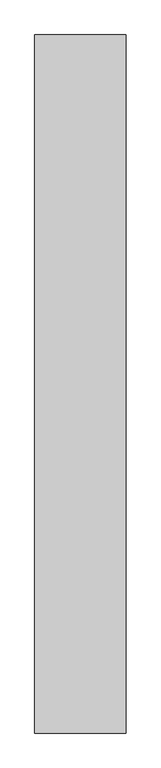
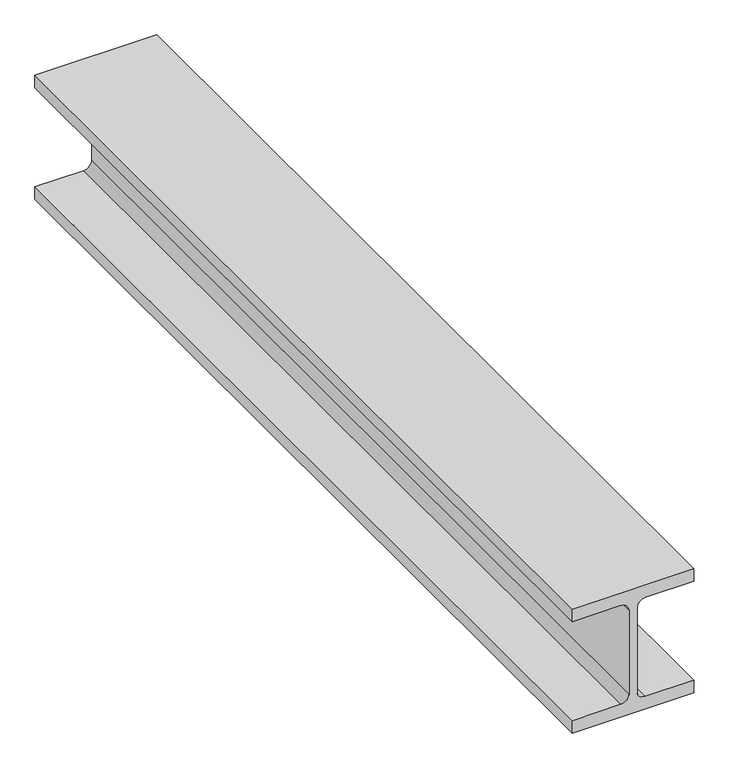
"""IFC4 building model written with IfcOpenShell, lengths in millimetres: proxy geometry, Structure061 17491 : Structure061 17491."""

import ifcopenshell
import ifcopenshell.guid

model = None  # the IFC model being written
_history = None  # IfcOwnerHistory: only IFC2X3 demands one
_inside = {}  # id of a spatial element -> (the spatial element, [elements in it])
_under = {}  # id of a project, library or spatial element -> (it, [spatial elements below it])
_declared = {}  # id of a project -> (the project, [libraries it declares])
_typed = {}  # id of a type object -> (the type object, [elements of that type])
_made_of = {}  # id of a material, layer set ... -> (it, [elements and type objects made of it])


def new_model(schema):
    """Start an empty IFC model of exactly this schema.

    Asked for "IFC4X3", IfcOpenShell would pick the latest addendum, in which some entities
    have other attributes; the version numbers below select the first issue.
    IFC2X3 requires an IfcOwnerHistory on every rooted entity: one is made here for all.
    """
    global model, _history
    if schema == "IFC4X3":
        model = ifcopenshell.file(schema_version=(4, 3, 0, 0))
    else:
        model = ifcopenshell.file(schema=schema)
    _inside.clear()
    _under.clear()
    _declared.clear()
    _typed.clear()
    _made_of.clear()
    _history = None
    if model.schema == "IFC2X3":
        org = make("IfcOrganization", Name="unknown")
        user = make(
            "IfcPersonAndOrganization",
            ThePerson=make("IfcPerson", FamilyName="unknown"),
            TheOrganization=org,
        )
        app = make(
            "IfcApplication",
            ApplicationDeveloper=org,
            Version="unknown",
            ApplicationFullName="unknown",
            ApplicationIdentifier="unknown",
        )
        _history = make(
            "IfcOwnerHistory",
            OwningUser=user,
            OwningApplication=app,
            ChangeAction="ADDED",
            CreationDate=0,
        )
    return model


def make(cls, **values):
    """One entity of the class cls with the attributes given. An attribute that is None is left unset."""
    return model.create_entity(
        cls, **{name: value for name, value in values.items() if value is not None}
    )


def rooted(cls, **values):
    """An entity with a GlobalId (a new one), such as an element, a storey or a relation."""
    return make(cls, GlobalId=ifcopenshell.guid.new(), OwnerHistory=_history, **values)


def si_unit(unit_type, name, prefix=None):
    """IfcSIUnit, for example si_unit("LENGTHUNIT", "METRE", prefix="MILLI")."""
    return make("IfcSIUnit", UnitType=unit_type, Prefix=prefix, Name=name)


def assignment(units):
    """IfcUnitAssignment: the units of a project."""
    return None if units is None else make("IfcUnitAssignment", Units=units)


def point(xyz):
    """IfcCartesianPoint."""
    return None if xyz is None else make("IfcCartesianPoint", Coordinates=xyz)


def direction(xyz):
    """IfcDirection."""
    return None if xyz is None else make("IfcDirection", DirectionRatios=xyz)


def frame(location, z_axis=None, x_axis=None):
    """IfcAxis2Placement3D, a coordinate frame: its origin and axes. An axis left out is left unset."""
    return make(
        "IfcAxis2Placement3D",
        Location=point(location),
        Axis=direction(z_axis),
        RefDirection=direction(x_axis),
    )


def frame_2d(location, x_axis=None):
    """IfcAxis2Placement2D, a coordinate frame in the plane: its origin and x axis."""
    return make(
        "IfcAxis2Placement2D", Location=point(location), RefDirection=direction(x_axis)
    )


def origin():
    """The frame at (0, 0, 0) with its axes left unset."""
    return frame((0.0, 0.0, 0.0))


def place(relative_to, where):
    """IfcLocalPlacement: puts the frame where relative to a parent placement (None: the world)."""
    return make(
        "IfcLocalPlacement", PlacementRelTo=relative_to, RelativePlacement=where
    )


def context(
    kind, dimensions, precision=None, world=None, true_north=None, identifier=None
):
    """IfcGeometricRepresentationContext, for example the 3D "Model" context."""
    return make(
        "IfcGeometricRepresentationContext",
        ContextIdentifier=identifier,
        ContextType=kind,
        CoordinateSpaceDimension=dimensions,
        Precision=precision,
        WorldCoordinateSystem=world,
        TrueNorth=true_north,
    )


def project(units=None, contexts=None):
    """IfcProject with its units and contexts."""
    return rooted(
        "IfcProject",
        Name="project",
        RepresentationContexts=contexts,
        UnitsInContext=assignment(units),
    )


def spatial(cls, under=None, at=None, **own):
    """A site, building, storey or space (cls), placed at a placement, below another one or the project."""
    s = rooted(cls, ObjectPlacement=at, **own)
    if under is not None:
        _under.setdefault(under.id(), (under, []))[1].append(s)
    return s


def polyline(points):
    """IfcPolyline through the points."""
    return make("IfcPolyline", Points=[point(p) for p in points])


def circle_curve(where, radius):
    """IfcCircle in the frame where."""
    return make("IfcCircle", Position=where, Radius=radius)


def trimmed(basis, trim1, trim2, sense, master):
    """IfcTrimmedCurve: the piece of a basis curve between two trims."""
    return make(
        "IfcTrimmedCurve",
        BasisCurve=basis,
        Trim1=trim1,
        Trim2=trim2,
        SenseAgreement=sense,
        MasterRepresentation=master,
    )


def segment(curve, same_sense, transition):
    """IfcCompositeCurveSegment."""
    return make(
        "IfcCompositeCurveSegment",
        Transition=transition,
        SameSense=same_sense,
        ParentCurve=curve,
    )


def composite_curve(segments, self_intersect=None):
    """IfcCompositeCurve: segments joined end to end."""
    return make("IfcCompositeCurve", Segments=segments, SelfIntersect=self_intersect)


def outline(outer, holes=None, kind="AREA"):
    """IfcArbitraryClosedProfileDef: a profile drawn as a closed curve; with holes, ...WithVoids."""
    if holes is None:
        return make("IfcArbitraryClosedProfileDef", ProfileType=kind, OuterCurve=outer)
    return make(
        "IfcArbitraryProfileDefWithVoids",
        ProfileType=kind,
        OuterCurve=outer,
        InnerCurves=holes,
    )


def extrude(swept, where, along, depth):
    """IfcExtrudedAreaSolid: the profile swept, set in the frame where, extruded along a direction by depth."""
    return make(
        "IfcExtrudedAreaSolid",
        SweptArea=swept,
        Position=where,
        ExtrudedDirection=direction(along),
        Depth=depth,
    )


def shape(context_of_items, identifier, shape_type, items):
    """IfcShapeRepresentation: the items that make up one representation, for example the "Body"."""
    return make(
        "IfcShapeRepresentation",
        ContextOfItems=context_of_items,
        RepresentationIdentifier=identifier,
        RepresentationType=shape_type,
        Items=items,
    )


def source(mapping_origin, context_of_items, identifier, shape_type, items):
    """IfcRepresentationMap: a shape defined once, which mapped items show again and again."""
    return make(
        "IfcRepresentationMap",
        MappingOrigin=mapping_origin,
        MappedRepresentation=shape(context_of_items, identifier, shape_type, items),
    )


def transform(
    local_origin,
    x_axis=None,
    y_axis=None,
    z_axis=None,
    scale=None,
    scale2=None,
    scale3=None,
    uniform=True,
):
    """IfcCartesianTransformationOperator3D, or its non-uniform kind. x_axis, y_axis, z_axis: its Axis1, 2, 3."""
    if uniform:
        return make(
            "IfcCartesianTransformationOperator3D",
            Axis1=direction(x_axis),
            Axis2=direction(y_axis),
            LocalOrigin=point(local_origin),
            Scale=scale,
            Axis3=direction(z_axis),
        )
    return make(
        "IfcCartesianTransformationOperator3DnonUniform",
        Axis1=direction(x_axis),
        Axis2=direction(y_axis),
        LocalOrigin=point(local_origin),
        Scale=scale,
        Axis3=direction(z_axis),
        Scale2=scale2,
        Scale3=scale3,
    )


def mapped(mapping_source, mapping_target):
    """IfcMappedItem: shows the shape of a source again, moved by a transform."""
    return make(
        "IfcMappedItem", MappingSource=mapping_source, MappingTarget=mapping_target
    )


def made_of(thing, what):
    """Note that an element or type object is made of a material, layer set ...; save() writes the relation."""
    if what is not None:
        _made_of.setdefault(what.id(), (what, []))[1].append(thing)
    return thing


def element(
    cls,
    number,
    at=None,
    inside=None,
    cuts=None,
    type_object=None,
    material=None,
    context=None,
    identifier="Body",
    shape_type=None,
    held_by="IfcProductDefinitionShape",
    body=None,
    shapes=None,
    **own,
):
    """One element of the class cls, such as IfcWall. Its Tag is "e" and its number.

    at: its placement. inside: the storey or other place that contains it. cuts: it is an
    opening in that element (IfcRelVoidsElement). A single representation is given by context,
    identifier, shape_type and body (its items); several are given by shapes. held_by: the class
    of the entity that holds the representations. save() writes the other relations.
    """
    e = rooted(cls, Tag="e%d" % number, ObjectPlacement=at, **own)
    if body is not None:
        shapes = [shape(context, identifier, shape_type, body)]
    if shapes is not None:
        e.Representation = make(held_by, Representations=shapes)
    if inside is not None:
        _inside.setdefault(inside.id(), (inside, []))[1].append(e)
    if cuts is not None:
        rooted(
            "IfcRelVoidsElement", RelatingBuildingElement=cuts, RelatedOpeningElement=e
        )
    if type_object is not None:
        _typed.setdefault(type_object.id(), (type_object, []))[1].append(e)
    return made_of(e, material)


def aggregate(whole, parts):
    """IfcRelAggregates: a whole, such as a stair, and the parts it consists of."""
    return rooted("IfcRelAggregates", RelatingObject=whole, RelatedObjects=parts)


def save(model, path):
    """Write the relations noted so far, then the file.

    IfcRelAggregates (storeys below a building ...), IfcRelContainedInSpatialStructure (elements
    in a storey), IfcRelDefinesByType, IfcRelAssociatesMaterial and IfcRelDeclares: one each for
    every whole, place, type object, material and project.
    """
    for whole, parts in _under.values():
        aggregate(whole, parts)
    for where, things in _inside.values():
        rooted(
            "IfcRelContainedInSpatialStructure",
            RelatedElements=things,
            RelatingStructure=where,
        )
    for kind, things in _typed.values():
        rooted("IfcRelDefinesByType", RelatedObjects=things, RelatingType=kind)
    for what, things in _made_of.values():
        rooted("IfcRelAssociatesMaterial", RelatedObjects=things, RelatingMaterial=what)
    for by, libraries in _declared.values():
        rooted("IfcRelDeclares", RelatingContext=by, RelatedDefinitions=libraries)
    model.write(path)


def generic_models_2eef4193(model_context):
    return source(origin(), model_context, "Body", "SweptSolid", [
        extrude(outline(composite_curve([segment(trimmed(circle_curve(frame_2d((40003.1585, 7375.6117048)), 17.5895), [point((40003.1585, 7358.0222048))], [point((40020.748, 7375.6117048))], True, "CARTESIAN"), True, "CONTINUOUS"), segment(polyline([(40020.748, 7375.6117048), (40020.748, 7480.1962048), (40049.196, 7480.1962048), (40049.196, 7218.5762048), (40020.748, 7218.5762048), (40020.748, 7323.1607048)]), True, "CONTINUOUS"), segment(trimmed(circle_curve(frame_2d((40003.1585, 7323.1607048)), 17.5895), [point((40020.748, 7323.1607048))], [point((40003.1585, 7340.7502048))], True, "CARTESIAN"), True, "CONTINUOUS"), segment(polyline([(40003.1585, 7340.7502048), (39813.2935, 7340.7502048)]), True, "CONTINUOUS"), segment(trimmed(circle_curve(frame_2d((39813.2935, 7323.1607048)), 17.5895), [point((39813.2935, 7340.7502048))], [point((39795.704, 7323.1607048))], True, "CARTESIAN"), True, "CONTINUOUS"), segment(polyline([(39795.704, 7323.1607048), (39795.704, 7218.5762048), (39767.256, 7218.5762048), (39767.256, 7480.1962048), (39795.704, 7480.1962048), (39795.704, 7375.6117048)]), True, "CONTINUOUS"), segment(trimmed(circle_curve(frame_2d((39813.2935, 7375.6117048)), 17.5895), [point((39795.704, 7375.6117048))], [point((39813.2935, 7358.0222048))], True, "CARTESIAN"), True, "CONTINUOUS"), segment(polyline([(39813.2935, 7358.0222048), (40003.1585, 7358.0222048)]), True, "CONTINUOUS")], self_intersect=False)), frame((0.0, -3747.9491938, 0.0), z_axis=(0.0, 1.0, 0.0), x_axis=(0.0, 0.0, 1.0)), (0.0, 0.0, 1.0), 2000.0),
    ])


if __name__ == "__main__":
    model = new_model("IFC4")
    model_context = context("Model", 3, world=origin())
    ifc_project = project(units=[si_unit("LENGTHUNIT", "METRE", prefix="MILLI")], contexts=[model_context])
    site = spatial("IfcSite", under=ifc_project)
    building = spatial("IfcBuilding", under=site)
    placement = place(None, origin())
    generic_models_shape = generic_models_2eef4193(model_context)
    element("IfcBuildingElementProxy", 1, Name="Structure061 17491 : Structure061 17491", ObjectType="Structure061 17491 : Structure061 17491", at=placement, inside=building, context=model_context, shape_type="MappedRepresentation", body=[
        mapped(generic_models_shape, transform((0.0, 0.0, 0.0), x_axis=(1.0, 0.0, 0.0), y_axis=(0.0, 1.0, 0.0), z_axis=(0.0, 0.0, 1.0))),
    ])
    save(model, "model.ifc")

# Revit data of these elements
# Type "Structure061 17491 : Structure061 17491"
#   NameOverride = "Structure061"
# Element 1 (IfcBuildingElementProxy, "Structure061 17491 : Structure061 17491")
#   Materials on its faces: "STEEL STRUCTURE (SEE STRUCTURAL DWGS)"
# Materials
#   "STEEL STRUCTURE (SEE STRUCTURAL DWGS)": class "Unassigned", colour RGB 128 128 128, transparency 0, Cost = 0
